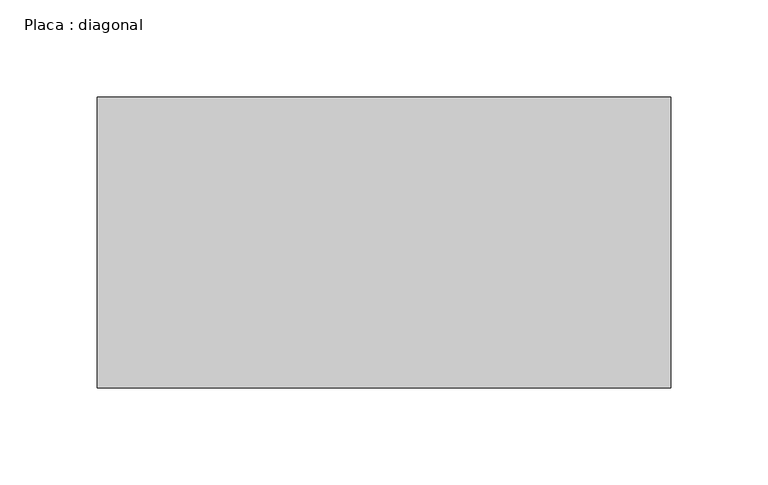
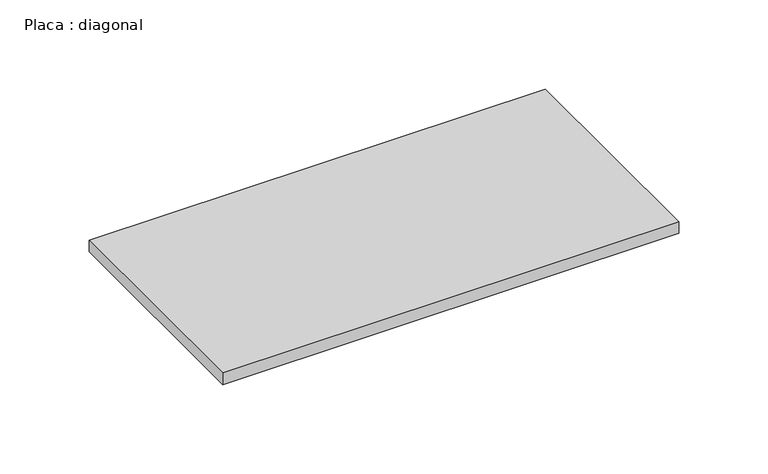
"""IFC4 building model written with IfcOpenShell, lengths in millimetres: beam geometry, Placa : diagonal."""

from ifc_helpers import new_model, si_unit, frame, origin, place, context, project, spatial, polyline, outline, extrude, source, transform, mapped, element, save


def placa_diagonal_32176e84(model_context):
    return source(origin(), model_context, "Body", "SweptSolid", [
        extrude(outline(polyline([(148.4670022, 75.0), (148.4670022, -75.0), (-147.3519629, -75.0), (-147.3519629, 75.0), (148.4670022, 75.0)])), frame((0.0, 0.0, -4.0), z_axis=(0.0, 0.0, 1.0), x_axis=(1.0, 0.0, 0.0)), (0.0, 0.0, 1.0), 8.0),
    ])


if __name__ == "__main__":
    model = new_model("IFC4")
    model_context = context("Model", 3, world=origin())
    ifc_project = project(units=[si_unit("LENGTHUNIT", "METRE", prefix="MILLI")], contexts=[model_context])
    site = spatial("IfcSite", under=ifc_project)
    building = spatial("IfcBuilding", under=site)
    placement = place(None, origin())
    placa_diagonal_shape = placa_diagonal_32176e84(model_context)
    element("IfcBeam", 1, ObjectType="Placa : diagonal", at=placement, inside=building, context=model_context, shape_type="MappedRepresentation", body=[
        mapped(placa_diagonal_shape, transform((0.0, 0.0, 0.0), x_axis=(1.0, 0.0, 0.0), y_axis=(0.0, 1.0, 0.0), z_axis=(0.0, 0.0, 1.0))),
    ])
    save(model, "model.ifc")

# Revit data of these elements
# Type "Placa : diagonal"
#   W = 0
#   Length [instance default] = 1.50 m
#   b = 0.15 m
#   d = 0.008 m
#   A = 0 m²
#   Structural Material [instance default] = Aço, 45-345
# Element 1 (IfcBeam, "Placa : diagonal")
#   Materials on its faces: "Aço, 45-345"
# Materials
#   "Aço, 45-345": class "Metal", colour RGB 247 247 247, transparency 0, Description = "Aço 345 MPa", Cost = 0
